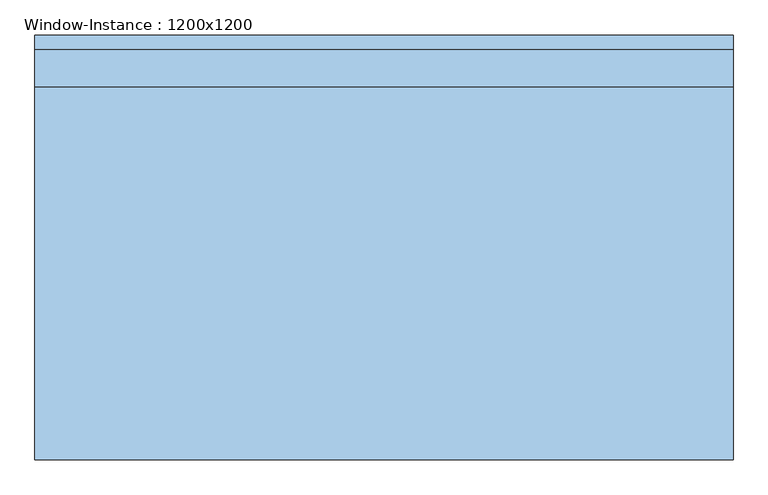
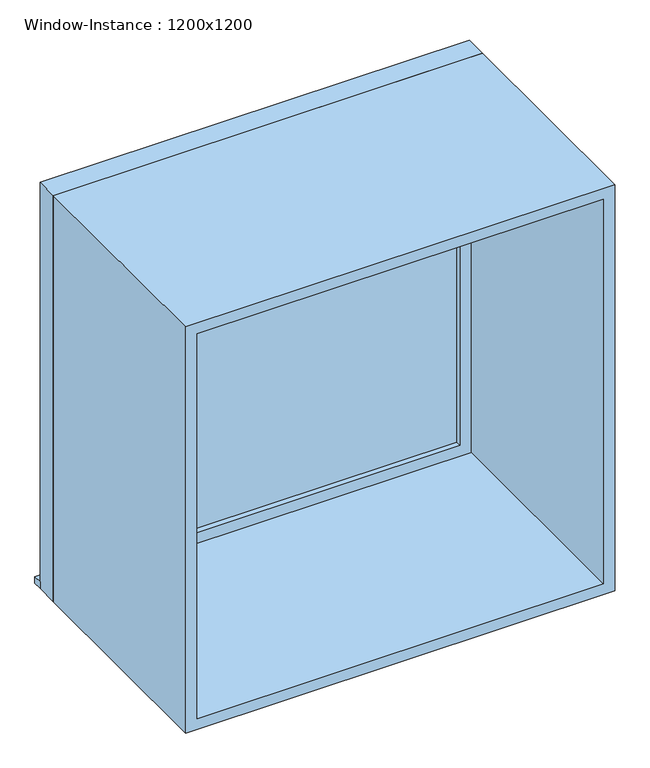
"""IFC4 building model written with IfcOpenShell, lengths in millimetres: window geometry, Window-Instance : 1200x1200."""

from ifc_helpers import new_model, si_unit, frame, origin, place, context, project, spatial, polyline, outline, extrude, source, transform, mapped, element, save


def window_instance_1200x1200_01b7a31e(model_context):
    return source(origin(), model_context, "Body", "SweptSolid", [
        extrude(outline(polyline([(-638.1, 377.9), (561.9, 377.9), (561.9, 352.5), (-638.1, 352.5), (-638.1, 377.9)])), frame((0.0, 0.0, 900.0), z_axis=(0.0, 0.0, 1.0), x_axis=(1.0, 0.0, 0.0)), (0.0, 0.0, 1.0), 19.05),
        extrude(outline(polyline([(498.4, 303.925), (-574.6, 303.925), (-574.6, 316.625), (498.4, 316.625), (498.4, 303.925)])), frame((0.0, 0.0, 963.5), z_axis=(0.0, 0.0, 1.0), x_axis=(1.0, 0.0, 0.0)), (0.0, 0.0, 1.0), 1073.0),
        extrude(outline(polyline([(2080.95, -619.05), (919.05, -619.05), (919.05, 542.85), (2080.95, 542.85), (2080.95, -619.05)]), holes=[polyline([(2036.5, -574.6), (2036.5, 498.4), (963.5, 498.4), (963.5, -574.6), (2036.5, -574.6)])]), frame((0.0, 288.05, 0.0), z_axis=(0.0, 1.0, 0.0), x_axis=(0.0, 0.0, 1.0)), (0.0, 0.0, 1.0), 44.45),
        extrude(outline(polyline([(2100.0, -638.1), (900.0, -638.1), (900.0, 561.9), (2100.0, 561.9), (2100.0, -638.1)]), holes=[polyline([(2068.25, -606.35), (2068.25, 530.15), (931.75, 530.15), (931.75, -606.35), (2068.25, -606.35)])]), frame((0.0, -352.5, 0.0), z_axis=(0.0, 1.0, 0.0), x_axis=(0.0, 0.0, 1.0)), (0.0, 0.0, 1.0), 640.55),
        extrude(outline(polyline([(2100.0, 561.9), (2100.0, -638.1), (900.0, -638.1), (900.0, 561.9), (2100.0, 561.9)]), holes=[polyline([(2080.95, 542.85), (919.05, 542.85), (919.05, -619.05), (2080.95, -619.05), (2080.95, 542.85)])]), frame((0.0, 288.05, 0.0), z_axis=(0.0, 1.0, 0.0), x_axis=(0.0, 0.0, 1.0)), (0.0, 0.0, 1.0), 64.45),
    ])


if __name__ == "__main__":
    model = new_model("IFC4")
    model_context = context("Model", 3, world=origin())
    ifc_project = project(units=[si_unit("LENGTHUNIT", "METRE", prefix="MILLI")], contexts=[model_context])
    site = spatial("IfcSite", under=ifc_project)
    building = spatial("IfcBuilding", under=site)
    placement = place(None, origin())
    window_instance_1200x1200_shape = window_instance_1200x1200_01b7a31e(model_context)
    element("IfcWindow", 1, ObjectType="Window-Instance : 1200x1200", at=placement, inside=building, context=model_context, shape_type="MappedRepresentation", body=[
        mapped(window_instance_1200x1200_shape, transform((0.0, 0.0, 0.0), x_axis=(1.0, 0.0, 0.0), y_axis=(0.0, 1.0, 0.0), z_axis=(0.0, 0.0, 1.0))),
    ])
    save(model, "model.ifc")

# Revit data of these elements
# Type "Window-Instance : 1200x1200"
#   Type Mark = "11"
#   Construction Type Id = "GSP4R"
#   Assembly Code = "B2020100"
#   Analytic Construction = "1/8 in Pilkington single glazing"
#   Visual Light Transmittance = 0.9
#   Thermal Resistance (R) = 0.149095 (m²·K)/W
#   Solar Heat Gain Coefficient = 0.86
#   Heat Transfer Coefficient (U) = 6.70716 W/(m²·K)
#   Height [instance default] = 1200 mm
#   Default Sill Height = 900 mm
#   Width [instance default] = 600 mm
#   Window Inset = 20 mm
#   Glass Pane Material = none
#   Sash Material = none
#   Wall Closure = (empty or 0)
# Element 1 (IfcWindow, "Window-Instance : 1200x1200")
#   Width = 1200 mm
